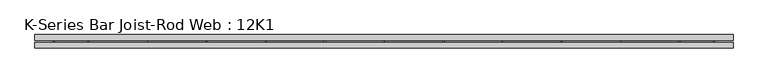
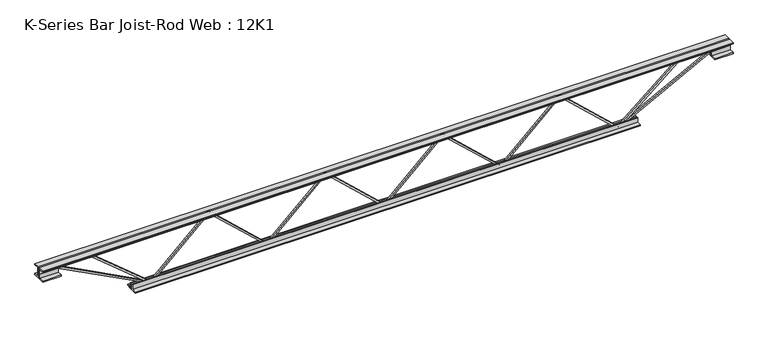
"""IFC4 building model written with IfcOpenShell, lengths in millimetres: beam geometry, K-Series Bar Joist-Rod Web : 12K1."""

from ifc_helpers import new_model, si_unit, frame, origin, place, context, project, spatial, polyline, outline, extrude, source, transform, mapped, element, save


def k_series_bar_joist_rod_web_12k1_8b3ada06(model_context):
    return source(origin(), model_context, "Body", "SweptSolid", [
        extrude(outline(polyline([(-141.2875, 0.0), (-150.8125, 0.0), (-150.8125, 5.0462518), (141.2875, 319.3712518), (141.2875, 321.9787482), (-150.8125, 636.3037482), (-150.8125, 641.35), (-141.2875, 641.35), (-141.2875, 640.0462518), (150.8125, 325.7212518), (150.8125, 315.6287482), (-141.2875, 1.3037482), (-141.2875, 0.0)])), frame((0.0, -4.7625, 0.0), z_axis=(0.0, 1.0, 0.0), x_axis=(0.0, 0.0, 1.0)), (0.0, 0.0, 1.0), 9.525),
        extrude(outline(polyline([(-141.2875, -641.35), (-150.8125, -641.35), (-150.8125, -636.3037482), (141.2875, -321.9787482), (141.2875, -319.3712518), (-150.8125, -5.0462518), (-150.8125, 0.0), (-141.2875, 0.0), (-141.2875, -1.3037482), (150.8125, -315.6287482), (150.8125, -325.7212518), (-141.2875, -640.0462518), (-141.2875, -641.35)])), frame((0.0, -4.7625, 0.0), z_axis=(0.0, 1.0, 0.0), x_axis=(0.0, 0.0, 1.0)), (0.0, 0.0, 1.0), 9.525),
        extrude(outline(polyline([(-141.2875, 641.35), (-150.8125, 641.35), (-150.8125, 646.3962518), (141.2875, 960.7212518), (141.2875, 963.3287482), (-150.8125, 1277.6537482), (-150.8125, 1282.7), (-141.2875, 1282.7), (-141.2875, 1281.3962518), (150.8125, 967.0712518), (150.8125, 956.9787482), (-141.2875, 642.6537482), (-141.2875, 641.35)])), frame((0.0, -4.7625, 0.0), z_axis=(0.0, 1.0, 0.0), x_axis=(0.0, 0.0, 1.0)), (0.0, 0.0, 1.0), 9.525),
        extrude(outline(polyline([(-141.2875, -1282.7), (-150.8125, -1282.7), (-150.8125, -1277.6537482), (141.2875, -963.3287482), (141.2875, -960.7212518), (-150.8125, -646.3962518), (-150.8125, -641.35), (-141.2875, -641.35), (-141.2875, -642.6537482), (150.8125, -956.9787482), (150.8125, -967.0712518), (-141.2875, -1281.3962518), (-141.2875, -1282.7)])), frame((0.0, -4.7625, 0.0), z_axis=(0.0, 1.0, 0.0), x_axis=(0.0, 0.0, 1.0)), (0.0, 0.0, 1.0), 9.525),
        extrude(outline(polyline([(4.7625, 152.4), (36.5125, 152.4), (36.5125, 146.05), (11.1125, 146.05), (11.1125, 120.65), (4.7625, 120.65), (4.7625, 152.4)])), frame((-1892.3, 0.0, 0.0), z_axis=(1.0, 0.0, 0.0), x_axis=(0.0, 1.0, 0.0)), (0.0, 0.0, 1.0), 3784.6),
        extrude(outline(polyline([(-4.7625, 152.4), (-4.7625, 120.65), (-11.1125, 120.65), (-11.1125, 146.05), (-36.5125, 146.05), (-36.5125, 152.4), (-4.7625, 152.4)])), frame((-1892.3, 0.0, 0.0), z_axis=(1.0, 0.0, 0.0), x_axis=(0.0, 1.0, 0.0)), (0.0, 0.0, 1.0), 3784.6),
        extrude(outline(polyline([(-4.7625, 88.9), (-36.5125, 88.9), (-36.5125, 95.25), (-11.1125, 95.25), (-11.1125, 120.65), (-4.7625, 120.65), (-4.7625, 88.9)])), frame((-1892.3, 0.0, 0.0), z_axis=(1.0, 0.0, 0.0), x_axis=(0.0, 1.0, 0.0)), (0.0, 0.0, 1.0), 101.6),
        extrude(outline(polyline([(36.5125, 88.9), (4.7625, 88.9), (4.7625, 120.65), (11.1125, 120.65), (11.1125, 95.25), (36.5125, 95.25), (36.5125, 88.9)])), frame((-1892.3, 0.0, 0.0), z_axis=(1.0, 0.0, 0.0), x_axis=(0.0, 1.0, 0.0)), (0.0, 0.0, 1.0), 101.6),
        extrude(outline(polyline([(4.7625, 88.9), (4.7625, 120.65), (11.1125, 120.65), (11.1125, 95.25), (36.5125, 95.25), (36.5125, 88.9), (4.7625, 88.9)])), frame((1790.7, 0.0, 0.0), z_axis=(1.0, 0.0, 0.0), x_axis=(0.0, 1.0, 0.0)), (0.0, 0.0, 1.0), 101.6),
        extrude(outline(polyline([(-4.7625, 88.9), (-36.5125, 88.9), (-36.5125, 95.25), (-11.1125, 95.25), (-11.1125, 120.65), (-4.7625, 120.65), (-4.7625, 88.9)])), frame((1790.7, 0.0, 0.0), z_axis=(1.0, 0.0, 0.0), x_axis=(0.0, 1.0, 0.0)), (0.0, 0.0, 1.0), 101.6),
        extrude(outline(polyline([(4.7625, -152.4), (4.7625, -120.65), (11.1125, -120.65), (11.1125, -146.05), (36.5125, -146.05), (36.5125, -152.4), (4.7625, -152.4)])), frame((-1384.3, 0.0, 0.0), z_axis=(1.0, 0.0, 0.0), x_axis=(0.0, 1.0, 0.0)), (0.0, 0.0, 1.0), 2768.6),
        extrude(outline(polyline([(-4.7625, -152.4), (-36.5125, -152.4), (-36.5125, -146.05), (-11.1125, -146.05), (-11.1125, -120.65), (-4.7625, -120.65), (-4.7625, -152.4)])), frame((-1384.3, 0.0, 0.0), z_axis=(1.0, 0.0, 0.0), x_axis=(0.0, 1.0, 0.0)), (0.0, 0.0, 1.0), 2768.6),
        extrude(outline(polyline([(0.0, -9.525), (0.0, 0.0), (573.7533355, 0.0), (573.7533355, -9.525), (0.0, -9.525)])), frame((-1792.9137714, 4.7625, 116.4332925), z_axis=(0.464833898989514, 0.0, 0.885397902838157), x_axis=(0.885397902838157, 0.0, -0.464833898989514)), (0.0, 0.0, 1.0), 9.525),
        extrude(outline(polyline([(0.0, -9.525), (0.0, 0.0), (417.0867363, 0.0), (417.0867363, -9.525), (0.0, -9.525)])), frame((-1606.4203108, 4.7625, 116.9883763), z_axis=(0.6394353422613703, 0.0, 0.768844875815066), x_axis=(0.768844875815066, 0.0, -0.6394353422613703)), (0.0, 0.0, 1.0), 9.525),
        extrude(outline(polyline([(0.0, -9.525), (0.0, 0.0), (573.7533355, 0.0), (573.7533355, -9.525), (0.0, -9.525)])), frame((1792.9137714, -4.7625, 116.4332925), z_axis=(-0.4648338989894953, 0.0, 0.8853979028381667), x_axis=(-0.8853979028381667, 0.0, -0.4648338989894953)), (0.0, 0.0, 1.0), 9.525),
        extrude(outline(polyline([(0.0, -9.525), (0.0, 0.0), (417.0867363, 0.0), (417.0867363, -9.525), (0.0, -9.525)])), frame((1606.4203108, -4.7625, 116.9883763), z_axis=(-0.639435342261365, 0.0, 0.7688448758150705), x_axis=(-0.7688448758150705, 0.0, -0.639435342261365)), (0.0, 0.0, 1.0), 9.525),
    ])


if __name__ == "__main__":
    model = new_model("IFC4")
    model_context = context("Model", 3, world=origin())
    ifc_project = project(units=[si_unit("LENGTHUNIT", "METRE", prefix="MILLI")], contexts=[model_context])
    site = spatial("IfcSite", under=ifc_project)
    building = spatial("IfcBuilding", under=site)
    placement = place(None, origin())
    k_series_bar_joist_rod_web_12k1_shape = k_series_bar_joist_rod_web_12k1_8b3ada06(model_context)
    element("IfcBeam", 1, ObjectType="K-Series Bar Joist-Rod Web : 12K1", at=placement, inside=building, context=model_context, shape_type="MappedRepresentation", body=[
        mapped(k_series_bar_joist_rod_web_12k1_shape, transform((0.0, 0.0, 0.0), x_axis=(1.0, 0.0, 0.0), y_axis=(0.0, 1.0, 0.0), z_axis=(0.0, 0.0, 1.0))),
    ])
    save(model, "model.ifc")

# Revit data of these elements
# Type "K-Series Bar Joist-Rod Web : 12K1"
#   Assembly Code = "B1010350"
#   Wt = 5
#   Web Thickness = 0' - 0 3/8"
#   Start Offset [instance default] = 0' - 0"
#   Start Extension [instance default] = 0' - 0"
#   Seat Length = 0' - 4"
#   Seat Depth = 0' - 2 1/2"
#   PanelArrayLength [instance default] = 20' - 0"
#   Panel [instance default] = 2' - 0"
#   End Offset [instance default] = 0' - 0"
#   End Extension [instance default] = 0' - 0"
#   End Panel = 2' - 0"
#   Cord Leg = 0' - 1 1/4"
#   Chord Thickness = 0' - 0 1/4"
#   Length [instance default] = 24' - 0"
#   Depth = 1' - 0"
#   PanelArrayNum [instance default] = 10
#   Structural Material = none
# Element 1 (IfcBeam, "K-Series Bar Joist-Rod Web : 12K1")
#   PanelArrayLength = 8' - 5"
#   Panel = 2' - 1 1/4"
#   PanelArrayNum = 4
